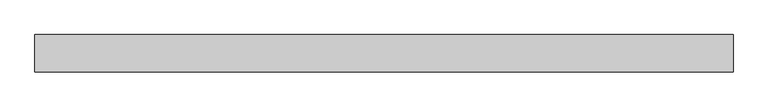
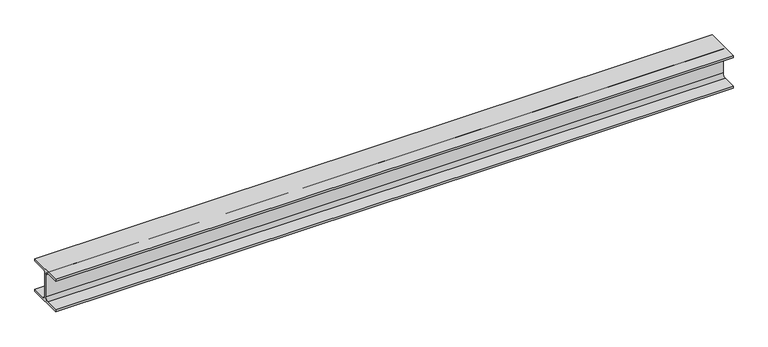
"""IFC4 building model written with IfcOpenShell, lengths in millimetres: beam geometry, NLRS_28_SF_LIB_stalen ligger HEA-AV-CWV-MMBS-SRP_gen_rsf : stalen ligger_gen__HEA 160."""

from ifc_helpers import new_model, si_unit, point, frame, frame_2d, origin, place, context, project, spatial, polyline, circle_curve, trimmed, segment, composite_curve, outline, extrude, source, transform, mapped, element, save


def beam_5e2477af(model_context):
    return source(origin(), model_context, "Body", "SweptSolid", [
        extrude(outline(composite_curve([segment(polyline([(80.0, 67.0), (18.0, 67.0)]), True, "CONTINUOUS"), segment(trimmed(circle_curve(frame_2d((18.0, 52.0)), 15.0), [point((18.0, 67.0))], [point((3.0, 52.0))], True, "CARTESIAN"), True, "CONTINUOUS"), segment(polyline([(3.0, 52.0), (3.0, -52.0)]), True, "CONTINUOUS"), segment(trimmed(circle_curve(frame_2d((18.0, -52.0)), 15.0), [point((3.0, -52.0))], [point((18.0, -67.0))], True, "CARTESIAN"), True, "CONTINUOUS"), segment(polyline([(18.0, -67.0), (80.0, -67.0), (80.0, -76.0), (-80.0, -76.0), (-80.0, -67.0), (-18.0, -67.0)]), True, "CONTINUOUS"), segment(trimmed(circle_curve(frame_2d((-18.0, -52.0)), 15.0), [point((-18.0, -67.0))], [point((-3.0, -52.0))], True, "CARTESIAN"), True, "CONTINUOUS"), segment(polyline([(-3.0, -52.0), (-3.0, 52.0)]), True, "CONTINUOUS"), segment(trimmed(circle_curve(frame_2d((-18.0, 52.0)), 15.0), [point((-3.0, 52.0))], [point((-18.0, 67.0))], True, "CARTESIAN"), True, "CONTINUOUS"), segment(polyline([(-18.0, 67.0), (-80.0, 67.0), (-80.0, 76.0), (80.0, 76.0), (80.0, 67.0)]), True, "CONTINUOUS")], self_intersect=False)), frame((-1499.9999994, 0.0, 0.0), z_axis=(1.0, 0.0, 0.0), x_axis=(0.0, 1.0, 0.0)), (0.0, 0.0, 1.0), 2999.9999988),
    ])


if __name__ == "__main__":
    model = new_model("IFC4")
    model_context = context("Model", 3, world=origin())
    ifc_project = project(units=[si_unit("LENGTHUNIT", "METRE", prefix="MILLI")], contexts=[model_context])
    site = spatial("IfcSite", under=ifc_project)
    building = spatial("IfcBuilding", under=site)
    placement = place(None, origin())
    beam_shape = beam_5e2477af(model_context)
    element("IfcBeam", 1, ObjectType="NLRS_28_SF_LIB_stalen ligger HEA-AV-CWV-MMBS-SRP_gen_rsf : stalen ligger_gen__HEA 160", at=placement, inside=building, context=model_context, shape_type="MappedRepresentation", body=[
        mapped(beam_shape, transform((0.0, 0.0, 0.0), x_axis=(1.0, 0.0, 0.0), y_axis=(0.0, 1.0, 0.0), z_axis=(0.0, 0.0, 1.0))),
    ])
    save(model, "model.ifc")

# Revit data of these elements
# Type "NLRS_28_SF_LIB_stalen ligger HEA-AV-CWV-MMBS-SRP_gen_rsf : stalen ligger_gen__HEA 160"
#   Type IfcGUID = "3PFmhy1jzBXho9jMrHR46u"
#   IfcExportAs = "IfcBeamType"
#   Type Comments = "HEA160"
#   Model = " "
#   Manufacturer = " "
#   Fire Rating = " "
#   Description = "stalen ligger HEA160"
#   Assembly Code = "28.11"
#   ra = 15 mm
#   vz = 76 mm
#   vy = 80 mm
#   vpz = 76 mm
#   vpy = 80 mm
#   NLRS_C_lengte [instance default] = 1500 mm
#   Length [instance default] = 1500 mm
#   bf = 160 mm
#   d = 152 mm
#   tf = 9 mm
#   tw = 6 mm
#   Structural Material = NLRS_h2_staal_gen_rsf
#   Keynote = ""
# Element 1 (IfcBeam, "NLRS_28_SF_LIB_stalen ligger HEA-AV-CWV-MMBS-SRP_gen_rsf : stalen ligger_gen__HEA 160")
#   NLRS_C_lengte = 3000 mm
#   Materials on its faces: "NLRS_h2_staal_gen_rsf"
# Materials
#   "NLRS_h2_staal_gen_rsf": class "H - Metaal", colour RGB 189 187 185, transparency 0, Keynote = "h2", Manufacturer = "Revit Standards Foundation", URL = "www.revitstandards.org", Description = "staal", Cost = 0
